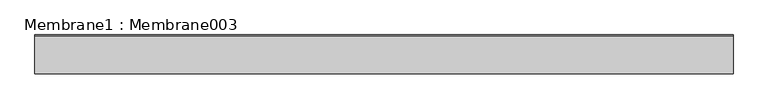
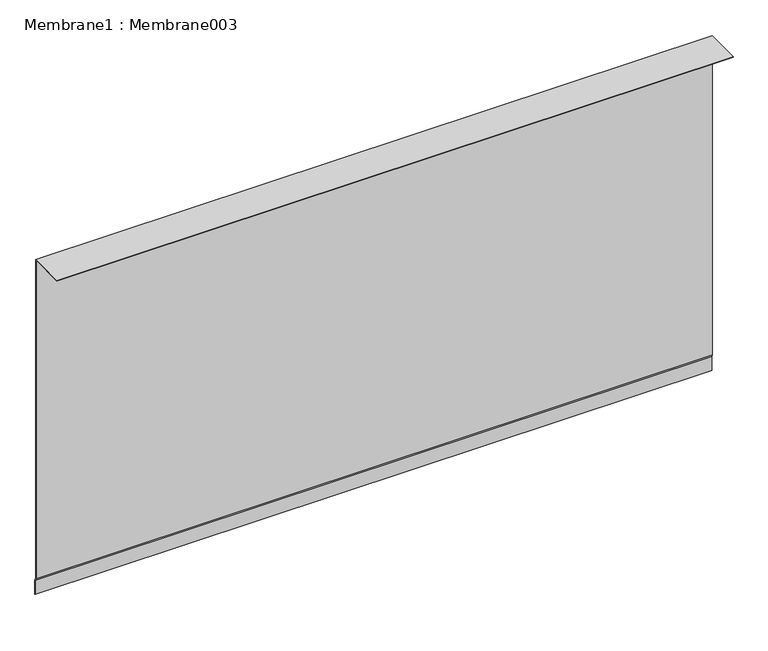
"""IFC4 building model written with IfcOpenShell, lengths in millimetres: proxy geometry, Membrane1 : Membrane003."""

from ifc_helpers import new_model, si_unit, frame, origin, place, context, project, spatial, polyline, outline, extrude, source, transform, mapped, element, save


def membrane1_membrane003_52707934(model_context):
    return source(origin(), model_context, "Body", "SweptSolid", [
        extrude(outline(polyline([(9754.8834401, 36494.0399441), (9750.723729, 36501.0477566), (9750.723729, 37497.8101563), (9644.9242604, 37497.8101563), (9644.9242604, 37499.3101563), (9752.223729, 37499.3101563), (9752.223729, 36501.4594133), (9756.3834401, 36494.4516008), (9756.3834401, 36450.0458609), (9754.8834401, 36450.0458609), (9754.8834401, 36494.0399441)])), frame((3694.2883192, 0.0, 0.0), z_axis=(1.0, 0.0, 0.0), x_axis=(0.0, 1.0, 0.0)), (0.0, 0.0, 1.0), 2000.0),
    ])


if __name__ == "__main__":
    model = new_model("IFC4")
    model_context = context("Model", 3, world=origin())
    ifc_project = project(units=[si_unit("LENGTHUNIT", "METRE", prefix="MILLI")], contexts=[model_context])
    site = spatial("IfcSite", under=ifc_project)
    building = spatial("IfcBuilding", under=site)
    placement = place(None, origin())
    membrane1_membrane003_shape = membrane1_membrane003_52707934(model_context)
    element("IfcBuildingElementProxy", 1, Name="Membrane1 : Membrane003", ObjectType="Membrane1 : Membrane003", at=placement, inside=building, context=model_context, shape_type="MappedRepresentation", body=[
        mapped(membrane1_membrane003_shape, transform((0.0, 0.0, 0.0), x_axis=(1.0, 0.0, 0.0), y_axis=(0.0, 1.0, 0.0), z_axis=(0.0, 0.0, 1.0))),
    ])
    save(model, "model.ifc")

# Revit data of these elements
# Type "Membrane1 : Membrane003"
#   NameOverride = "Membrane003"
# Element 1 (IfcBuildingElementProxy, "Membrane1 : Membrane003")
#   Materials on its faces: "(2) LAYERS OF ICE & WATER SHIELD (BITUTHANE) UNDER STUCCO"
# Materials
#   "(2) LAYERS OF ICE & WATER SHIELD (BITUTHANE) UNDER STUCCO": class "Unassigned", colour RGB 186 255 159, transparency 0, Cost = 0
